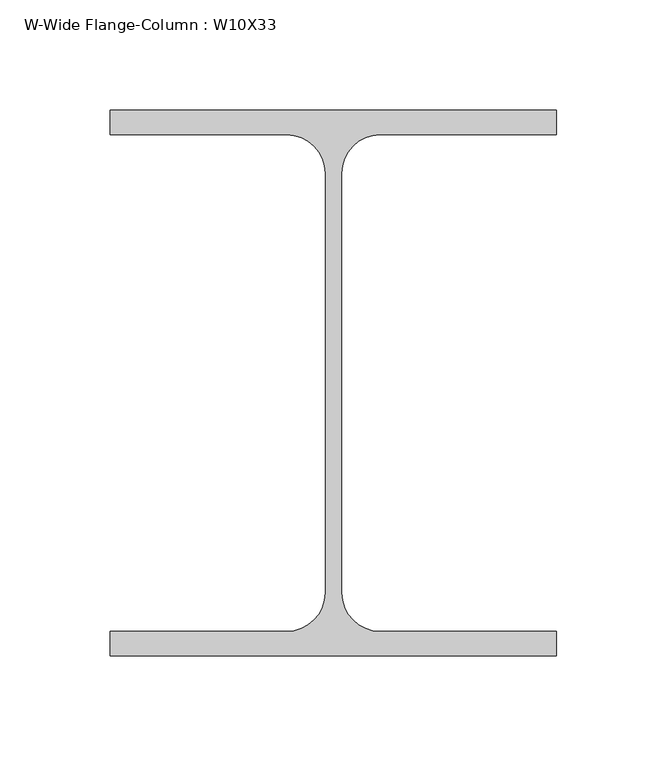
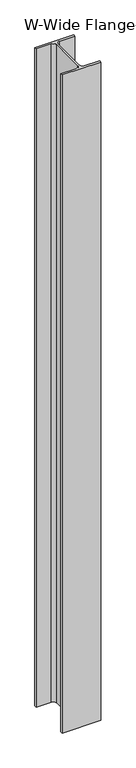
"""IFC4 building model written with IfcOpenShell, lengths in millimetres: column geometry, W-Wide Flange-Column : W10X33."""

import ifcopenshell
import ifcopenshell.guid

model = None  # the IFC model being written
_history = None  # IfcOwnerHistory: only IFC2X3 demands one
_inside = {}  # id of a spatial element -> (the spatial element, [elements in it])
_under = {}  # id of a project, library or spatial element -> (it, [spatial elements below it])
_declared = {}  # id of a project -> (the project, [libraries it declares])
_typed = {}  # id of a type object -> (the type object, [elements of that type])
_made_of = {}  # id of a material, layer set ... -> (it, [elements and type objects made of it])


def new_model(schema):
    """Start an empty IFC model of exactly this schema.

    Asked for "IFC4X3", IfcOpenShell would pick the latest addendum, in which some entities
    have other attributes; the version numbers below select the first issue.
    IFC2X3 requires an IfcOwnerHistory on every rooted entity: one is made here for all.
    """
    global model, _history
    if schema == "IFC4X3":
        model = ifcopenshell.file(schema_version=(4, 3, 0, 0))
    else:
        model = ifcopenshell.file(schema=schema)
    _inside.clear()
    _under.clear()
    _declared.clear()
    _typed.clear()
    _made_of.clear()
    _history = None
    if model.schema == "IFC2X3":
        org = make("IfcOrganization", Name="unknown")
        user = make(
            "IfcPersonAndOrganization",
            ThePerson=make("IfcPerson", FamilyName="unknown"),
            TheOrganization=org,
        )
        app = make(
            "IfcApplication",
            ApplicationDeveloper=org,
            Version="unknown",
            ApplicationFullName="unknown",
            ApplicationIdentifier="unknown",
        )
        _history = make(
            "IfcOwnerHistory",
            OwningUser=user,
            OwningApplication=app,
            ChangeAction="ADDED",
            CreationDate=0,
        )
    return model


def make(cls, **values):
    """One entity of the class cls with the attributes given. An attribute that is None is left unset."""
    return model.create_entity(
        cls, **{name: value for name, value in values.items() if value is not None}
    )


def rooted(cls, **values):
    """An entity with a GlobalId (a new one), such as an element, a storey or a relation."""
    return make(cls, GlobalId=ifcopenshell.guid.new(), OwnerHistory=_history, **values)


def si_unit(unit_type, name, prefix=None):
    """IfcSIUnit, for example si_unit("LENGTHUNIT", "METRE", prefix="MILLI")."""
    return make("IfcSIUnit", UnitType=unit_type, Prefix=prefix, Name=name)


def assignment(units):
    """IfcUnitAssignment: the units of a project."""
    return None if units is None else make("IfcUnitAssignment", Units=units)


def point(xyz):
    """IfcCartesianPoint."""
    return None if xyz is None else make("IfcCartesianPoint", Coordinates=xyz)


def direction(xyz):
    """IfcDirection."""
    return None if xyz is None else make("IfcDirection", DirectionRatios=xyz)


def frame(location, z_axis=None, x_axis=None):
    """IfcAxis2Placement3D, a coordinate frame: its origin and axes. An axis left out is left unset."""
    return make(
        "IfcAxis2Placement3D",
        Location=point(location),
        Axis=direction(z_axis),
        RefDirection=direction(x_axis),
    )


def frame_2d(location, x_axis=None):
    """IfcAxis2Placement2D, a coordinate frame in the plane: its origin and x axis."""
    return make(
        "IfcAxis2Placement2D", Location=point(location), RefDirection=direction(x_axis)
    )


def origin():
    """The frame at (0, 0, 0) with its axes left unset."""
    return frame((0.0, 0.0, 0.0))


def place(relative_to, where):
    """IfcLocalPlacement: puts the frame where relative to a parent placement (None: the world)."""
    return make(
        "IfcLocalPlacement", PlacementRelTo=relative_to, RelativePlacement=where
    )


def context(
    kind, dimensions, precision=None, world=None, true_north=None, identifier=None
):
    """IfcGeometricRepresentationContext, for example the 3D "Model" context."""
    return make(
        "IfcGeometricRepresentationContext",
        ContextIdentifier=identifier,
        ContextType=kind,
        CoordinateSpaceDimension=dimensions,
        Precision=precision,
        WorldCoordinateSystem=world,
        TrueNorth=true_north,
    )


def project(units=None, contexts=None):
    """IfcProject with its units and contexts."""
    return rooted(
        "IfcProject",
        Name="project",
        RepresentationContexts=contexts,
        UnitsInContext=assignment(units),
    )


def spatial(cls, under=None, at=None, **own):
    """A site, building, storey or space (cls), placed at a placement, below another one or the project."""
    s = rooted(cls, ObjectPlacement=at, **own)
    if under is not None:
        _under.setdefault(under.id(), (under, []))[1].append(s)
    return s


def polyline(points):
    """IfcPolyline through the points."""
    return make("IfcPolyline", Points=[point(p) for p in points])


def circle_curve(where, radius):
    """IfcCircle in the frame where."""
    return make("IfcCircle", Position=where, Radius=radius)


def trimmed(basis, trim1, trim2, sense, master):
    """IfcTrimmedCurve: the piece of a basis curve between two trims."""
    return make(
        "IfcTrimmedCurve",
        BasisCurve=basis,
        Trim1=trim1,
        Trim2=trim2,
        SenseAgreement=sense,
        MasterRepresentation=master,
    )


def segment(curve, same_sense, transition):
    """IfcCompositeCurveSegment."""
    return make(
        "IfcCompositeCurveSegment",
        Transition=transition,
        SameSense=same_sense,
        ParentCurve=curve,
    )


def composite_curve(segments, self_intersect=None):
    """IfcCompositeCurve: segments joined end to end."""
    return make("IfcCompositeCurve", Segments=segments, SelfIntersect=self_intersect)


def outline(outer, holes=None, kind="AREA"):
    """IfcArbitraryClosedProfileDef: a profile drawn as a closed curve; with holes, ...WithVoids."""
    if holes is None:
        return make("IfcArbitraryClosedProfileDef", ProfileType=kind, OuterCurve=outer)
    return make(
        "IfcArbitraryProfileDefWithVoids",
        ProfileType=kind,
        OuterCurve=outer,
        InnerCurves=holes,
    )


def extrude(swept, where, along, depth):
    """IfcExtrudedAreaSolid: the profile swept, set in the frame where, extruded along a direction by depth."""
    return make(
        "IfcExtrudedAreaSolid",
        SweptArea=swept,
        Position=where,
        ExtrudedDirection=direction(along),
        Depth=depth,
    )


def shape(context_of_items, identifier, shape_type, items):
    """IfcShapeRepresentation: the items that make up one representation, for example the "Body"."""
    return make(
        "IfcShapeRepresentation",
        ContextOfItems=context_of_items,
        RepresentationIdentifier=identifier,
        RepresentationType=shape_type,
        Items=items,
    )


def source(mapping_origin, context_of_items, identifier, shape_type, items):
    """IfcRepresentationMap: a shape defined once, which mapped items show again and again."""
    return make(
        "IfcRepresentationMap",
        MappingOrigin=mapping_origin,
        MappedRepresentation=shape(context_of_items, identifier, shape_type, items),
    )


def transform(
    local_origin,
    x_axis=None,
    y_axis=None,
    z_axis=None,
    scale=None,
    scale2=None,
    scale3=None,
    uniform=True,
):
    """IfcCartesianTransformationOperator3D, or its non-uniform kind. x_axis, y_axis, z_axis: its Axis1, 2, 3."""
    if uniform:
        return make(
            "IfcCartesianTransformationOperator3D",
            Axis1=direction(x_axis),
            Axis2=direction(y_axis),
            LocalOrigin=point(local_origin),
            Scale=scale,
            Axis3=direction(z_axis),
        )
    return make(
        "IfcCartesianTransformationOperator3DnonUniform",
        Axis1=direction(x_axis),
        Axis2=direction(y_axis),
        LocalOrigin=point(local_origin),
        Scale=scale,
        Axis3=direction(z_axis),
        Scale2=scale2,
        Scale3=scale3,
    )


def mapped(mapping_source, mapping_target):
    """IfcMappedItem: shows the shape of a source again, moved by a transform."""
    return make(
        "IfcMappedItem", MappingSource=mapping_source, MappingTarget=mapping_target
    )


def made_of(thing, what):
    """Note that an element or type object is made of a material, layer set ...; save() writes the relation."""
    if what is not None:
        _made_of.setdefault(what.id(), (what, []))[1].append(thing)
    return thing


def element(
    cls,
    number,
    at=None,
    inside=None,
    cuts=None,
    type_object=None,
    material=None,
    context=None,
    identifier="Body",
    shape_type=None,
    held_by="IfcProductDefinitionShape",
    body=None,
    shapes=None,
    **own,
):
    """One element of the class cls, such as IfcWall. Its Tag is "e" and its number.

    at: its placement. inside: the storey or other place that contains it. cuts: it is an
    opening in that element (IfcRelVoidsElement). A single representation is given by context,
    identifier, shape_type and body (its items); several are given by shapes. held_by: the class
    of the entity that holds the representations. save() writes the other relations.
    """
    e = rooted(cls, Tag="e%d" % number, ObjectPlacement=at, **own)
    if body is not None:
        shapes = [shape(context, identifier, shape_type, body)]
    if shapes is not None:
        e.Representation = make(held_by, Representations=shapes)
    if inside is not None:
        _inside.setdefault(inside.id(), (inside, []))[1].append(e)
    if cuts is not None:
        rooted(
            "IfcRelVoidsElement", RelatingBuildingElement=cuts, RelatedOpeningElement=e
        )
    if type_object is not None:
        _typed.setdefault(type_object.id(), (type_object, []))[1].append(e)
    return made_of(e, material)


def aggregate(whole, parts):
    """IfcRelAggregates: a whole, such as a stair, and the parts it consists of."""
    return rooted("IfcRelAggregates", RelatingObject=whole, RelatedObjects=parts)


def save(model, path):
    """Write the relations noted so far, then the file.

    IfcRelAggregates (storeys below a building ...), IfcRelContainedInSpatialStructure (elements
    in a storey), IfcRelDefinesByType, IfcRelAssociatesMaterial and IfcRelDeclares: one each for
    every whole, place, type object, material and project.
    """
    for whole, parts in _under.values():
        aggregate(whole, parts)
    for where, things in _inside.values():
        rooted(
            "IfcRelContainedInSpatialStructure",
            RelatedElements=things,
            RelatingStructure=where,
        )
    for kind, things in _typed.values():
        rooted("IfcRelDefinesByType", RelatedObjects=things, RelatingType=kind)
    for what, things in _made_of.values():
        rooted("IfcRelAssociatesMaterial", RelatedObjects=things, RelatingMaterial=what)
    for by, libraries in _declared.values():
        rooted("IfcRelDeclares", RelatingContext=by, RelatedDefinitions=libraries)
    model.write(path)


def w_wide_flange_column_w10x33_4909dbaa(model_context):
    return source(origin(), model_context, "Body", "SweptSolid", [
        extrude(outline(composite_curve([segment(polyline([(101.092, 123.571), (101.092, 112.522), (21.209, 112.522)]), True, "CONTINUOUS"), segment(trimmed(circle_curve(frame_2d((21.209, 94.996)), 17.526), [point((21.209, 112.522))], [point((3.683, 94.996))], True, "CARTESIAN"), True, "CONTINUOUS"), segment(polyline([(3.683, 94.996), (3.683, -94.996)]), True, "CONTINUOUS"), segment(trimmed(circle_curve(frame_2d((21.209, -94.996)), 17.526), [point((3.683, -94.996))], [point((21.209, -112.522))], True, "CARTESIAN"), True, "CONTINUOUS"), segment(polyline([(21.209, -112.522), (101.092, -112.522), (101.092, -123.571), (-101.092, -123.571), (-101.092, -112.522), (-21.209, -112.522)]), True, "CONTINUOUS"), segment(trimmed(circle_curve(frame_2d((-21.209, -94.996)), 17.526), [point((-21.209, -112.522))], [point((-3.683, -94.996))], True, "CARTESIAN"), True, "CONTINUOUS"), segment(polyline([(-3.683, -94.996), (-3.683, 94.996)]), True, "CONTINUOUS"), segment(trimmed(circle_curve(frame_2d((-21.209, 94.996)), 17.526), [point((-3.683, 94.996))], [point((-21.209, 112.522))], True, "CARTESIAN"), True, "CONTINUOUS"), segment(polyline([(-21.209, 112.522), (-101.092, 112.522), (-101.092, 123.571), (101.092, 123.571)]), True, "CONTINUOUS")], self_intersect=False)), frame((0.0, 0.0, 12566.65), z_axis=(0.0, 0.0, 1.0), x_axis=(1.0, 0.0, 0.0)), (0.0, 0.0, 1.0), 3638.55),
    ])


if __name__ == "__main__":
    model = new_model("IFC4")
    model_context = context("Model", 3, world=origin())
    ifc_project = project(units=[si_unit("LENGTHUNIT", "METRE", prefix="MILLI")], contexts=[model_context])
    site = spatial("IfcSite", under=ifc_project)
    building = spatial("IfcBuilding", under=site)
    placement = place(None, origin())
    w_wide_flange_column_w10x33_shape = w_wide_flange_column_w10x33_4909dbaa(model_context)
    element("IfcColumn", 1, ObjectType="W-Wide Flange-Column : W10X33", at=placement, inside=building, context=model_context, shape_type="MappedRepresentation", body=[
        mapped(w_wide_flange_column_w10x33_shape, transform((0.0, 0.0, 0.0), x_axis=(1.0, 0.0, 0.0), y_axis=(0.0, 1.0, 0.0), z_axis=(0.0, 0.0, 1.0))),
    ])
    save(model, "model.ifc")

# Revit data of these elements
# Type "W-Wide Flange-Column : W10X33"
#   Assembly Code = "B10"
#   W = 33
#   bf = 0' - 7.96"
#   d = 0' - 9.73"
#   k = 0' - 1 1/8"
#   kr = 0' - 0.69"
#   tf = 0' - 0.435"
#   tw = 0' - 0.29"
#   A = 0.0674306 SF
#   Structural Material [instance default] = Steel ASTM A992
# Element 1 (IfcColumn, "W-Wide Flange-Column : W10X33")
#   Materials on its faces: "Steel ASTM A992"
# Materials
#   "Steel ASTM A992": class "Metal", colour RGB 199 199 199, transparency 0, Description = "Structural steel 50ksi", Cost = 0
